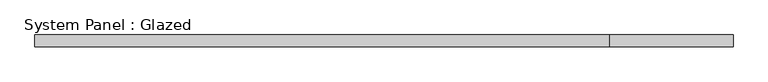
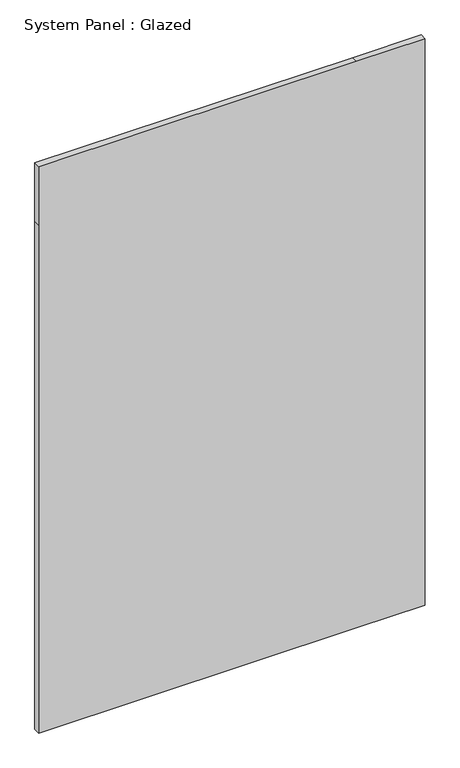
"""IFC4 building model written with IfcOpenShell, lengths in millimetres: plate geometry, System Panel : Glazed."""

from ifc_helpers import new_model, si_unit, frame, origin, place, context, project, spatial, polyline, outline, extrude, source, transform, mapped, element, save


def system_panel_glazed_8d3e4aee(model_context):
    return source(origin(), model_context, "Body", "SweptSolid", [
        extrude(outline(polyline([(0.0, -756.44375), (0.0, 488.95), (0.0, 756.44375), (2101.85, 756.44375), (2343.15, 756.44375), (2343.15, 488.95), (2343.15, -756.44375), (2101.85, -756.44375), (0.0, -756.44375)])), frame((0.0, -44.45, 0.0), z_axis=(0.0, 1.0, 0.0), x_axis=(0.0, 0.0, 1.0)), (0.0, 0.0, 1.0), 25.4),
    ])


if __name__ == "__main__":
    model = new_model("IFC4")
    model_context = context("Model", 3, world=origin())
    ifc_project = project(units=[si_unit("LENGTHUNIT", "METRE", prefix="MILLI")], contexts=[model_context])
    site = spatial("IfcSite", under=ifc_project)
    building = spatial("IfcBuilding", under=site)
    placement = place(None, origin())
    system_panel_glazed_shape = system_panel_glazed_8d3e4aee(model_context)
    element("IfcPlate", 1, ObjectType="System Panel : Glazed", at=placement, inside=building, context=model_context, shape_type="MappedRepresentation", body=[
        mapped(system_panel_glazed_shape, transform((0.0, 0.0, 0.0), x_axis=(1.0, 0.0, 0.0), y_axis=(0.0, 1.0, 0.0), z_axis=(0.0, 0.0, 1.0))),
    ])
    save(model, "model.ifc")

# Revit data of these elements
# Element 1 (IfcPlate, "System Panel : Glazed")
#   Materials on its faces: "Glass"
# Materials
#   "Glass": class "Glass", colour RGB 0 128 192, transparency 0.75
